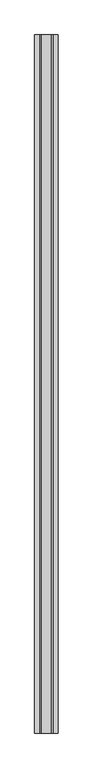
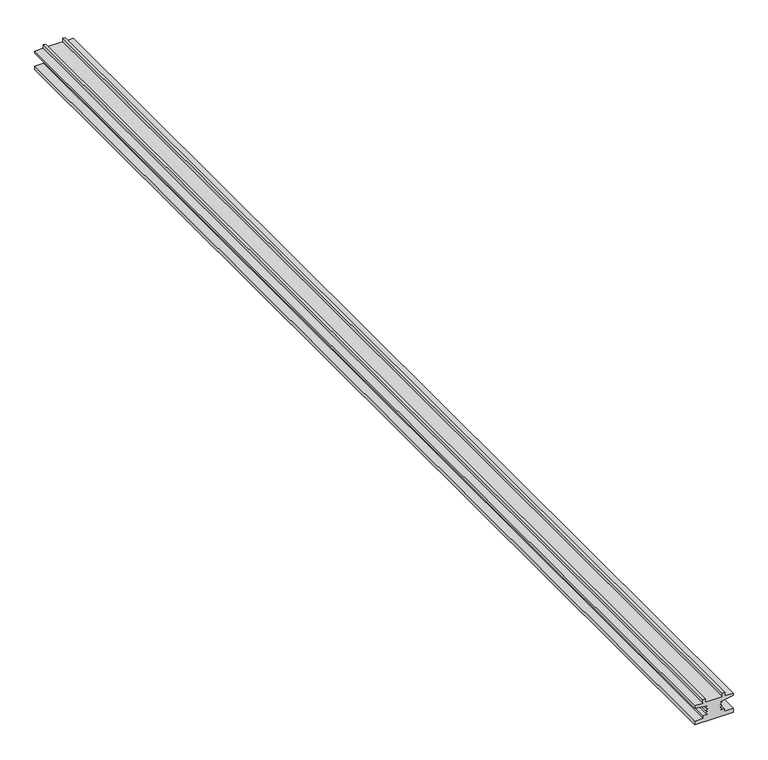
"""IFC4 building model written with IfcOpenShell, lengths in millimetres: proxy geometry, Bison pedestal1 : Bison pedestal004."""

import ifcopenshell
import ifcopenshell.guid

model = None  # the IFC model being written
_history = None  # IfcOwnerHistory: only IFC2X3 demands one
_inside = {}  # id of a spatial element -> (the spatial element, [elements in it])
_under = {}  # id of a project, library or spatial element -> (it, [spatial elements below it])
_declared = {}  # id of a project -> (the project, [libraries it declares])
_typed = {}  # id of a type object -> (the type object, [elements of that type])
_made_of = {}  # id of a material, layer set ... -> (it, [elements and type objects made of it])


def new_model(schema):
    """Start an empty IFC model of exactly this schema.

    Asked for "IFC4X3", IfcOpenShell would pick the latest addendum, in which some entities
    have other attributes; the version numbers below select the first issue.
    IFC2X3 requires an IfcOwnerHistory on every rooted entity: one is made here for all.
    """
    global model, _history
    if schema == "IFC4X3":
        model = ifcopenshell.file(schema_version=(4, 3, 0, 0))
    else:
        model = ifcopenshell.file(schema=schema)
    _inside.clear()
    _under.clear()
    _declared.clear()
    _typed.clear()
    _made_of.clear()
    _history = None
    if model.schema == "IFC2X3":
        org = make("IfcOrganization", Name="unknown")
        user = make(
            "IfcPersonAndOrganization",
            ThePerson=make("IfcPerson", FamilyName="unknown"),
            TheOrganization=org,
        )
        app = make(
            "IfcApplication",
            ApplicationDeveloper=org,
            Version="unknown",
            ApplicationFullName="unknown",
            ApplicationIdentifier="unknown",
        )
        _history = make(
            "IfcOwnerHistory",
            OwningUser=user,
            OwningApplication=app,
            ChangeAction="ADDED",
            CreationDate=0,
        )
    return model


def make(cls, **values):
    """One entity of the class cls with the attributes given. An attribute that is None is left unset."""
    return model.create_entity(
        cls, **{name: value for name, value in values.items() if value is not None}
    )


def rooted(cls, **values):
    """An entity with a GlobalId (a new one), such as an element, a storey or a relation."""
    return make(cls, GlobalId=ifcopenshell.guid.new(), OwnerHistory=_history, **values)


def si_unit(unit_type, name, prefix=None):
    """IfcSIUnit, for example si_unit("LENGTHUNIT", "METRE", prefix="MILLI")."""
    return make("IfcSIUnit", UnitType=unit_type, Prefix=prefix, Name=name)


def assignment(units):
    """IfcUnitAssignment: the units of a project."""
    return None if units is None else make("IfcUnitAssignment", Units=units)


def point(xyz):
    """IfcCartesianPoint."""
    return None if xyz is None else make("IfcCartesianPoint", Coordinates=xyz)


def direction(xyz):
    """IfcDirection."""
    return None if xyz is None else make("IfcDirection", DirectionRatios=xyz)


def frame(location, z_axis=None, x_axis=None):
    """IfcAxis2Placement3D, a coordinate frame: its origin and axes. An axis left out is left unset."""
    return make(
        "IfcAxis2Placement3D",
        Location=point(location),
        Axis=direction(z_axis),
        RefDirection=direction(x_axis),
    )


def origin():
    """The frame at (0, 0, 0) with its axes left unset."""
    return frame((0.0, 0.0, 0.0))


def place(relative_to, where):
    """IfcLocalPlacement: puts the frame where relative to a parent placement (None: the world)."""
    return make(
        "IfcLocalPlacement", PlacementRelTo=relative_to, RelativePlacement=where
    )


def context(
    kind, dimensions, precision=None, world=None, true_north=None, identifier=None
):
    """IfcGeometricRepresentationContext, for example the 3D "Model" context."""
    return make(
        "IfcGeometricRepresentationContext",
        ContextIdentifier=identifier,
        ContextType=kind,
        CoordinateSpaceDimension=dimensions,
        Precision=precision,
        WorldCoordinateSystem=world,
        TrueNorth=true_north,
    )


def project(units=None, contexts=None):
    """IfcProject with its units and contexts."""
    return rooted(
        "IfcProject",
        Name="project",
        RepresentationContexts=contexts,
        UnitsInContext=assignment(units),
    )


def spatial(cls, under=None, at=None, **own):
    """A site, building, storey or space (cls), placed at a placement, below another one or the project."""
    s = rooted(cls, ObjectPlacement=at, **own)
    if under is not None:
        _under.setdefault(under.id(), (under, []))[1].append(s)
    return s


def polyline(points):
    """IfcPolyline through the points."""
    return make("IfcPolyline", Points=[point(p) for p in points])


def outline(outer, holes=None, kind="AREA"):
    """IfcArbitraryClosedProfileDef: a profile drawn as a closed curve; with holes, ...WithVoids."""
    if holes is None:
        return make("IfcArbitraryClosedProfileDef", ProfileType=kind, OuterCurve=outer)
    return make(
        "IfcArbitraryProfileDefWithVoids",
        ProfileType=kind,
        OuterCurve=outer,
        InnerCurves=holes,
    )


def extrude(swept, where, along, depth):
    """IfcExtrudedAreaSolid: the profile swept, set in the frame where, extruded along a direction by depth."""
    return make(
        "IfcExtrudedAreaSolid",
        SweptArea=swept,
        Position=where,
        ExtrudedDirection=direction(along),
        Depth=depth,
    )


def shape(context_of_items, identifier, shape_type, items):
    """IfcShapeRepresentation: the items that make up one representation, for example the "Body"."""
    return make(
        "IfcShapeRepresentation",
        ContextOfItems=context_of_items,
        RepresentationIdentifier=identifier,
        RepresentationType=shape_type,
        Items=items,
    )


def source(mapping_origin, context_of_items, identifier, shape_type, items):
    """IfcRepresentationMap: a shape defined once, which mapped items show again and again."""
    return make(
        "IfcRepresentationMap",
        MappingOrigin=mapping_origin,
        MappedRepresentation=shape(context_of_items, identifier, shape_type, items),
    )


def transform(
    local_origin,
    x_axis=None,
    y_axis=None,
    z_axis=None,
    scale=None,
    scale2=None,
    scale3=None,
    uniform=True,
):
    """IfcCartesianTransformationOperator3D, or its non-uniform kind. x_axis, y_axis, z_axis: its Axis1, 2, 3."""
    if uniform:
        return make(
            "IfcCartesianTransformationOperator3D",
            Axis1=direction(x_axis),
            Axis2=direction(y_axis),
            LocalOrigin=point(local_origin),
            Scale=scale,
            Axis3=direction(z_axis),
        )
    return make(
        "IfcCartesianTransformationOperator3DnonUniform",
        Axis1=direction(x_axis),
        Axis2=direction(y_axis),
        LocalOrigin=point(local_origin),
        Scale=scale,
        Axis3=direction(z_axis),
        Scale2=scale2,
        Scale3=scale3,
    )


def mapped(mapping_source, mapping_target):
    """IfcMappedItem: shows the shape of a source again, moved by a transform."""
    return make(
        "IfcMappedItem", MappingSource=mapping_source, MappingTarget=mapping_target
    )


def made_of(thing, what):
    """Note that an element or type object is made of a material, layer set ...; save() writes the relation."""
    if what is not None:
        _made_of.setdefault(what.id(), (what, []))[1].append(thing)
    return thing


def element(
    cls,
    number,
    at=None,
    inside=None,
    cuts=None,
    type_object=None,
    material=None,
    context=None,
    identifier="Body",
    shape_type=None,
    held_by="IfcProductDefinitionShape",
    body=None,
    shapes=None,
    **own,
):
    """One element of the class cls, such as IfcWall. Its Tag is "e" and its number.

    at: its placement. inside: the storey or other place that contains it. cuts: it is an
    opening in that element (IfcRelVoidsElement). A single representation is given by context,
    identifier, shape_type and body (its items); several are given by shapes. held_by: the class
    of the entity that holds the representations. save() writes the other relations.
    """
    e = rooted(cls, Tag="e%d" % number, ObjectPlacement=at, **own)
    if body is not None:
        shapes = [shape(context, identifier, shape_type, body)]
    if shapes is not None:
        e.Representation = make(held_by, Representations=shapes)
    if inside is not None:
        _inside.setdefault(inside.id(), (inside, []))[1].append(e)
    if cuts is not None:
        rooted(
            "IfcRelVoidsElement", RelatingBuildingElement=cuts, RelatedOpeningElement=e
        )
    if type_object is not None:
        _typed.setdefault(type_object.id(), (type_object, []))[1].append(e)
    return made_of(e, material)


def aggregate(whole, parts):
    """IfcRelAggregates: a whole, such as a stair, and the parts it consists of."""
    return rooted("IfcRelAggregates", RelatingObject=whole, RelatedObjects=parts)


def save(model, path):
    """Write the relations noted so far, then the file.

    IfcRelAggregates (storeys below a building ...), IfcRelContainedInSpatialStructure (elements
    in a storey), IfcRelDefinesByType, IfcRelAssociatesMaterial and IfcRelDeclares: one each for
    every whole, place, type object, material and project.
    """
    for whole, parts in _under.values():
        aggregate(whole, parts)
    for where, things in _inside.values():
        rooted(
            "IfcRelContainedInSpatialStructure",
            RelatedElements=things,
            RelatingStructure=where,
        )
    for kind, things in _typed.values():
        rooted("IfcRelDefinesByType", RelatedObjects=things, RelatingType=kind)
    for what, things in _made_of.values():
        rooted("IfcRelAssociatesMaterial", RelatedObjects=things, RelatingMaterial=what)
    for by, libraries in _declared.values():
        rooted("IfcRelDeclares", RelatingContext=by, RelatedDefinitions=libraries)
    model.write(path)


def generic_models_1fc90002(model_context):
    return source(origin(), model_context, "Body", "SweptSolid", [
        extrude(outline(polyline([(36480.0342739, -2743.0545525), (36486.734375, -2742.9899902), (36486.734375, -2758.4094238), (36491.2120625, -2758.4094238), (36491.2120625, -2766.5004883), (36494.1534688, -2762.9697266), (36496.7296406, -2766.2797852), (36499.4503438, -2762.7492676), (36502.0245625, -2766.1328125), (36504.5577656, -2762.5581055), (36507.1046406, -2765.7746582), (36510.9913594, -2742.9899902), (36515.1456563, -2742.9899902), (36515.1456563, -2757.7331543), (36521.3116719, -2757.7331543), (36521.3116719, -2761.619873), (36515.1456563, -2761.619873), (36515.1456563, -2791.9099121), (36521.3116719, -2791.9099121), (36521.3116719, -2795.7966309), (36515.1456563, -2795.7966309), (36515.1456563, -2810.5397949), (36510.9913594, -2810.5397949), (36507.1046406, -2787.755127), (36504.5577656, -2790.9716797), (36502.0245625, -2787.3969727), (36499.4503438, -2790.7805176), (36496.7296406, -2787.25), (36494.1534688, -2790.5600586), (36491.2120625, -2787.0292969), (36491.2120625, -2795.1203613), (36486.734375, -2795.1203613), (36486.734375, -2810.5397949), (36480.0342739, -2810.4752326), (36480.0342739, -2743.0545525)])), frame((0.0, 998.1570053, 0.0), z_axis=(0.0, 1.0, 0.0), x_axis=(0.0, 0.0, 1.0)), (0.0, 0.0, 1.0), 2000.0),
    ])


if __name__ == "__main__":
    model = new_model("IFC4")
    model_context = context("Model", 3, world=origin())
    ifc_project = project(units=[si_unit("LENGTHUNIT", "METRE", prefix="MILLI")], contexts=[model_context])
    site = spatial("IfcSite", under=ifc_project)
    building = spatial("IfcBuilding", under=site)
    placement = place(None, origin())
    generic_models_shape = generic_models_1fc90002(model_context)
    element("IfcBuildingElementProxy", 1, Name="Bison pedestal1 : Bison pedestal004", ObjectType="Bison pedestal1 : Bison pedestal004", at=placement, inside=building, context=model_context, shape_type="MappedRepresentation", body=[
        mapped(generic_models_shape, transform((0.0, 0.0, 0.0), x_axis=(1.0, 0.0, 0.0), y_axis=(0.0, 1.0, 0.0), z_axis=(0.0, 0.0, 1.0))),
    ])
    save(model, "model.ifc")

# Revit data of these elements
# Type "Bison pedestal1 : Bison pedestal004"
#   NameOverride = "Bison pedestal004"
# Element 1 (IfcBuildingElementProxy, "Bison pedestal1 : Bison pedestal004")
#   Materials on its faces: "BUZON PEDESTAL"
# Materials
#   "BUZON PEDESTAL": class "Unassigned", colour RGB 66 66 66, transparency 0
